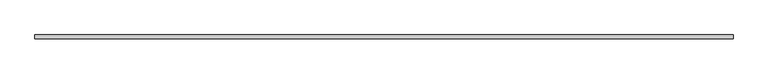
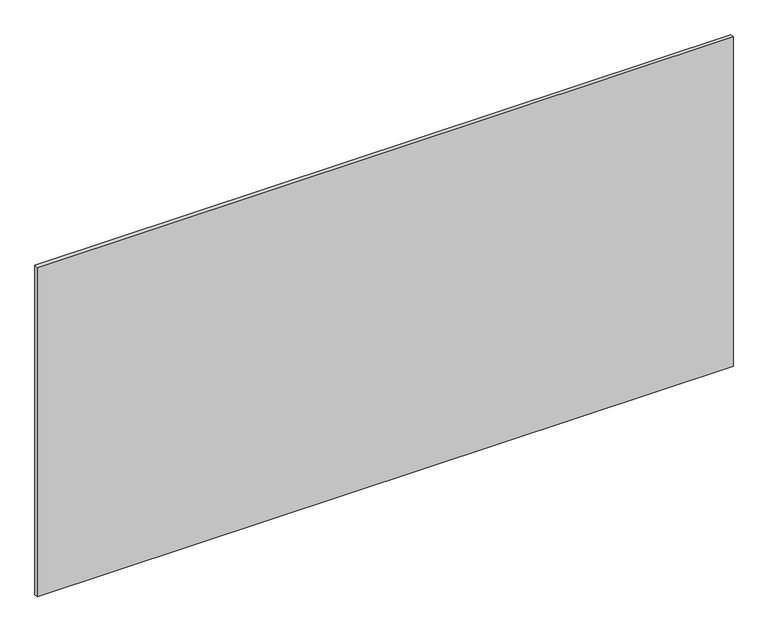
"""IFC4 building model written with IfcOpenShell, lengths in millimetres: proxy geometry, Inner panel:Inner panel:1:Inner panel:1 : Inner panel:Inner panel:300324:300043:Inner panel:1:Inner panel:1 : Inner panel:Inner panel:300324:300043 : Inner panel:Inner panel:1:Inner panel:1 : Inner panel:Inner panel:300324:300043:8 : Inner panel:Inner panel:1:Inner panel:1 : Inner panel:Inner panel:300324:300043:Inner panel:1:Inner panel:1 : Inner panel:Inner panel:300324:300043 : Inner panel:Inner panel:1:Inner panel:1 : Inner panel:Inner panel:300324:300043:300031."""

from ifc_helpers import new_model, si_unit, frame, origin, place, context, project, spatial, polyline, outline, extrude, source, transform, mapped, element, save


def generic_models_97f0f46e(model_context):
    return source(origin(), model_context, "Body", "SweptSolid", [
        extrude(outline(polyline([(570452.6367239, -579000.6913841), (572891.0367239, -579000.6913841), (572891.0367239, -579013.3913841), (570452.6367239, -579013.3913841), (570452.6367239, -579000.6913841)])), frame((0.0, 0.0, 2495.55), z_axis=(0.0, 0.0, 1.0), x_axis=(1.0, 0.0, 0.0)), (0.0, 0.0, 1.0), 1219.2),
    ])


if __name__ == "__main__":
    model = new_model("IFC4")
    model_context = context("Model", 3, world=origin())
    ifc_project = project(units=[si_unit("LENGTHUNIT", "METRE", prefix="MILLI")], contexts=[model_context])
    site = spatial("IfcSite", under=ifc_project)
    building = spatial("IfcBuilding", under=site)
    placement = place(None, origin())
    generic_models_shape = generic_models_97f0f46e(model_context)
    element("IfcBuildingElementProxy", 1, Name="Inner panel:Inner panel:1:Inner panel:1 : Inner panel:Inner panel:300324:300043:Inner panel:1:Inner panel:1 : Inner panel:Inner panel:300324:300043 : Inner panel:Inner panel:1:Inner panel:1 : Inner panel:Inner panel:300324:300043:8 : Inner panel:Inner panel:1:Inner panel:1 : Inner panel:Inner panel:300324:300043:Inner panel:1:Inner panel:1 : Inner panel:Inner panel:300324:300043 : Inner panel:Inner panel:1:Inner panel:1 : Inner panel:Inner panel:300324:300043:300031", ObjectType="Inner panel:Inner panel:1:Inner panel:1 : Inner panel:Inner panel:300324:300043:Inner panel:1:Inner panel:1 : Inner panel:Inner panel:300324:300043 : Inner panel:Inner panel:1:Inner panel:1 : Inner panel:Inner panel:300324:300043:8 : Inner panel:Inner panel:1:Inner panel:1 : Inner panel:Inner panel:300324:300043:Inner panel:1:Inner panel:1 : Inner panel:Inner panel:300324:300043 : Inner panel:Inner panel:1:Inner panel:1 : Inner panel:Inner panel:300324:300043:300031", at=placement, inside=building, context=model_context, shape_type="MappedRepresentation", body=[
        mapped(generic_models_shape, transform((0.0, 0.0, 0.0), x_axis=(1.0, 0.0, 0.0), y_axis=(0.0, 1.0, 0.0), z_axis=(0.0, 0.0, 1.0))),
    ])
    save(model, "model.ifc")

# Revit data of these elements
# Type "Inner panel:Inner panel:1:Inner panel:1 : Inner panel:Inner panel:300324:300043:Inner panel:1:Inner panel:1 : Inner panel:Inner panel:300324:300043 : Inner panel:Inner panel:1:Inner panel:1 : Inner panel:Inner panel:300324:300043:8 : Inner panel:Inner panel:1:Inner panel:1 : Inner panel:Inner panel:300324:300043:Inner panel:1:Inner panel:1 : Inner panel:Inner panel:300324:300043 : Inner panel:Inner panel:1:Inner panel:1 : Inner panel:Inner panel:300324:300043:300031"
#   NameOverride = "Inner panel:Inner panel:1:Inner panel:1 : Inner panel:Inner panel:300324:300043:Inner panel:1:Inner panel:1 : Inner panel:Inner panel:300324:300043 : Inner panel:Inner panel:1:Inner panel:1 : Inner panel:Inner panel:300324:300043:300031"
#   ObjectTypeOverride = "Inner panel:1:Inner panel:1 : Inner panel:Inner panel:300324:300043 : Inner panel:Inner panel:1:Inner panel:1 : Inner panel:Inner panel:300324:300043"
#   Reference = "Inner panel"
#   Tag = "300031"
# Element 1 (IfcBuildingElementProxy, "Inner panel:Inner panel:1:Inner panel:1 : Inner panel:Inner panel:300324:300043:Inner panel:1:Inner panel:1 : Inner panel:Inner panel:300324:300043 : Inner panel:Inner panel:1:Inner panel:1 : Inner panel:Inner panel:300324:300043:8 : Inner panel:Inner panel:1:Inner panel:1 : Inner panel:Inner panel:300324:300043:Inner panel:1:Inner panel:1 : Inner panel:Inner panel:300324:300043 : Inner panel:Inner panel:1:Inner panel:1 : Inner panel:Inner panel:300324:300043:300031")
#   Materials on its faces: "1/2\" EXTERIOR GRADE FIRE RETARDANT CDX PLYWOOD"
# Materials
#   "1/2\" EXTERIOR GRADE FIRE RETARDANT CDX PLYWOOD": class "Unassigned", colour RGB 196 177 123, transparency 0, Cost = 0
